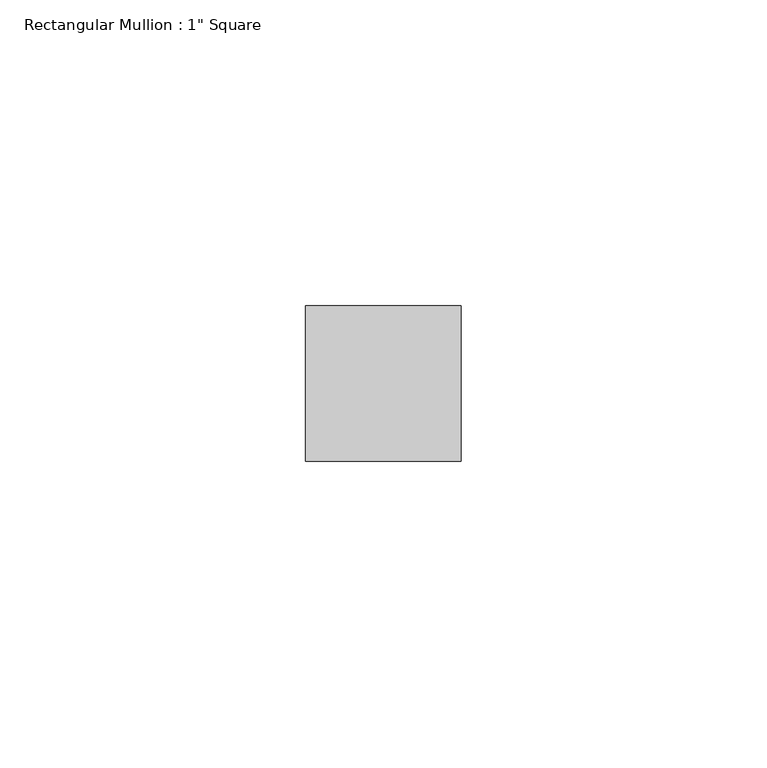
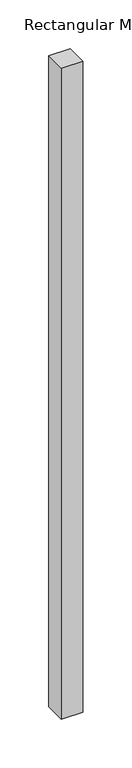
"""IFC4 building model written with IfcOpenShell, lengths in millimetres: member geometry."""

from ifc_helpers import new_model, si_unit, frame, origin, place, context, project, spatial, polyline, outline, extrude, source, transform, mapped, element, save


def member_efd737a5(model_context):
    return source(origin(), model_context, "Body", "SweptSolid", [
        extrude(outline(polyline([(12.7, 12.7), (12.7, -12.7), (-12.7, -12.7), (-12.7, 12.7), (12.7, 12.7)])), frame((0.0, 0.0, -812.8), z_axis=(0.0, 0.0, 1.0), x_axis=(1.0, 0.0, 0.0)), (0.0, 0.0, 1.0), 812.8),
    ])


if __name__ == "__main__":
    model = new_model("IFC4")
    model_context = context("Model", 3, world=origin())
    ifc_project = project(units=[si_unit("LENGTHUNIT", "METRE", prefix="MILLI")], contexts=[model_context])
    site = spatial("IfcSite", under=ifc_project)
    building = spatial("IfcBuilding", under=site)
    placement = place(None, origin())
    member_shape = member_efd737a5(model_context)
    element("IfcMember", 1, ObjectType="Rectangular Mullion : 1\" Square", at=placement, inside=building, context=model_context, shape_type="MappedRepresentation", body=[
        mapped(member_shape, transform((0.0, 0.0, 0.0), x_axis=(1.0, 0.0, 0.0), y_axis=(0.0, 1.0, 0.0), z_axis=(0.0, 0.0, 1.0))),
    ])
    save(model, "model.ifc")

# Revit data of these elements
# Type "Rectangular Mullion : 1\" Square"
#   built-in parameter 1007304 = 0.0833333 (stored number, unit not read)
#   built-in parameter 1007301 = 0.0416667 (stored number, unit not read)
#   built-in parameter 1007300 = 0.0416667 (stored number, unit not read)
# Element 1 (IfcMember, "Rectangular Mullion : 1\" Square")
#   Materials on its faces: "Metal - Aluminum"
# Materials
#   "Metal - Aluminum": class "Metal", colour RGB 247 247 247, transparency 0
